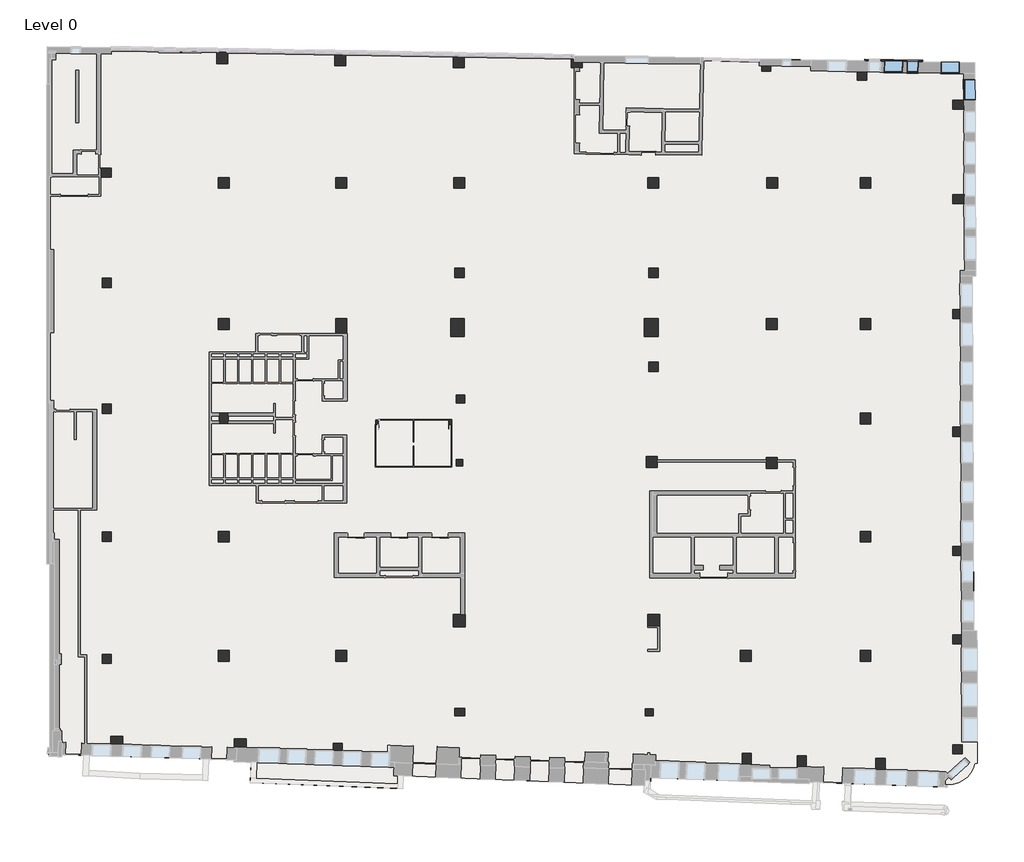
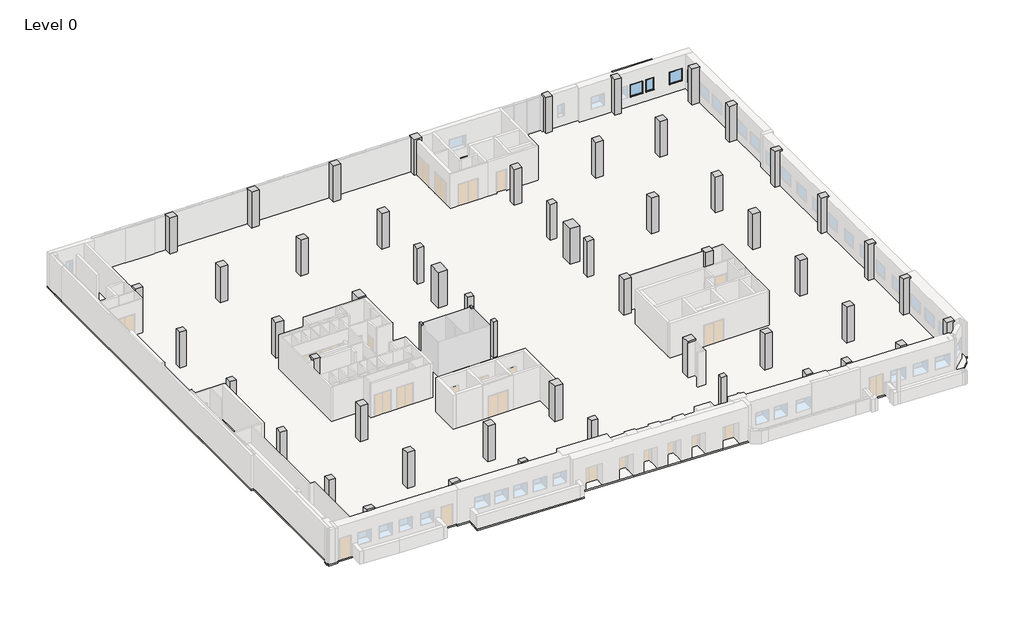
# One storey, part 9 of 9: 57 columns, 4 windows, 1 slab, 1 wall.
"""IFC4 building model written with IfcOpenShell, lengths in millimetres."""

import ifcopenshell
import ifcopenshell.guid

model = None  # the IFC model being written
_history = None  # IfcOwnerHistory: only IFC2X3 demands one
_inside = {}  # id of a spatial element -> (the spatial element, [elements in it])
_under = {}  # id of a project, library or spatial element -> (it, [spatial elements below it])
_declared = {}  # id of a project -> (the project, [libraries it declares])
_typed = {}  # id of a type object -> (the type object, [elements of that type])
_made_of = {}  # id of a material, layer set ... -> (it, [elements and type objects made of it])


def new_model(schema):
    """Start an empty IFC model of exactly this schema.

    Asked for "IFC4X3", IfcOpenShell would pick the latest addendum, in which some entities
    have other attributes; the version numbers below select the first issue.
    IFC2X3 requires an IfcOwnerHistory on every rooted entity: one is made here for all.
    """
    global model, _history
    if schema == "IFC4X3":
        model = ifcopenshell.file(schema_version=(4, 3, 0, 0))
    else:
        model = ifcopenshell.file(schema=schema)
    _inside.clear()
    _under.clear()
    _declared.clear()
    _typed.clear()
    _made_of.clear()
    _history = None
    if model.schema == "IFC2X3":
        org = make("IfcOrganization", Name="unknown")
        user = make(
            "IfcPersonAndOrganization",
            ThePerson=make("IfcPerson", FamilyName="unknown"),
            TheOrganization=org,
        )
        app = make(
            "IfcApplication",
            ApplicationDeveloper=org,
            Version="unknown",
            ApplicationFullName="unknown",
            ApplicationIdentifier="unknown",
        )
        _history = make(
            "IfcOwnerHistory",
            OwningUser=user,
            OwningApplication=app,
            ChangeAction="ADDED",
            CreationDate=0,
        )
    return model


def make(cls, **values):
    """One entity of the class cls with the attributes given. An attribute that is None is left unset."""
    return model.create_entity(
        cls, **{name: value for name, value in values.items() if value is not None}
    )


def rooted(cls, **values):
    """An entity with a GlobalId (a new one), such as an element, a storey or a relation."""
    return make(cls, GlobalId=ifcopenshell.guid.new(), OwnerHistory=_history, **values)


def si_unit(unit_type, name, prefix=None):
    """IfcSIUnit, for example si_unit("LENGTHUNIT", "METRE", prefix="MILLI")."""
    return make("IfcSIUnit", UnitType=unit_type, Prefix=prefix, Name=name)


def assignment(units):
    """IfcUnitAssignment: the units of a project."""
    return None if units is None else make("IfcUnitAssignment", Units=units)


def point(xyz):
    """IfcCartesianPoint."""
    return None if xyz is None else make("IfcCartesianPoint", Coordinates=xyz)


def direction(xyz):
    """IfcDirection."""
    return None if xyz is None else make("IfcDirection", DirectionRatios=xyz)


def frame(location, z_axis=None, x_axis=None):
    """IfcAxis2Placement3D, a coordinate frame: its origin and axes. An axis left out is left unset."""
    return make(
        "IfcAxis2Placement3D",
        Location=point(location),
        Axis=direction(z_axis),
        RefDirection=direction(x_axis),
    )


def frame_2d(location, x_axis=None):
    """IfcAxis2Placement2D, a coordinate frame in the plane: its origin and x axis."""
    return make(
        "IfcAxis2Placement2D", Location=point(location), RefDirection=direction(x_axis)
    )


def origin():
    """The frame at (0, 0, 0) with its axes left unset."""
    return frame((0.0, 0.0, 0.0))


def origin_with_axes():
    """The frame at (0, 0, 0) with the z axis (0, 0, 1) and the x axis (1, 0, 0) written out."""
    return frame((0.0, 0.0, 0.0), z_axis=(0.0, 0.0, 1.0), x_axis=(1.0, 0.0, 0.0))


def place(relative_to, where):
    """IfcLocalPlacement: puts the frame where relative to a parent placement (None: the world)."""
    return make(
        "IfcLocalPlacement", PlacementRelTo=relative_to, RelativePlacement=where
    )


def context(
    kind, dimensions, precision=None, world=None, true_north=None, identifier=None
):
    """IfcGeometricRepresentationContext, for example the 3D "Model" context."""
    return make(
        "IfcGeometricRepresentationContext",
        ContextIdentifier=identifier,
        ContextType=kind,
        CoordinateSpaceDimension=dimensions,
        Precision=precision,
        WorldCoordinateSystem=world,
        TrueNorth=true_north,
    )


def project(units=None, contexts=None):
    """IfcProject with its units and contexts."""
    return rooted(
        "IfcProject",
        Name="project",
        RepresentationContexts=contexts,
        UnitsInContext=assignment(units),
    )


def spatial(cls, under=None, at=None, **own):
    """A site, building, storey or space (cls), placed at a placement, below another one or the project."""
    s = rooted(cls, ObjectPlacement=at, **own)
    if under is not None:
        _under.setdefault(under.id(), (under, []))[1].append(s)
    return s


def polyline(points):
    """IfcPolyline through the points."""
    return make("IfcPolyline", Points=[point(p) for p in points])


def circle_curve(where, radius):
    """IfcCircle in the frame where."""
    return make("IfcCircle", Position=where, Radius=radius)


def trimmed(basis, trim1, trim2, sense, master):
    """IfcTrimmedCurve: the piece of a basis curve between two trims."""
    return make(
        "IfcTrimmedCurve",
        BasisCurve=basis,
        Trim1=trim1,
        Trim2=trim2,
        SenseAgreement=sense,
        MasterRepresentation=master,
    )


def segment(curve, same_sense, transition):
    """IfcCompositeCurveSegment."""
    return make(
        "IfcCompositeCurveSegment",
        Transition=transition,
        SameSense=same_sense,
        ParentCurve=curve,
    )


def composite_curve(segments, self_intersect=None):
    """IfcCompositeCurve: segments joined end to end."""
    return make("IfcCompositeCurve", Segments=segments, SelfIntersect=self_intersect)


def outline(outer, holes=None, kind="AREA"):
    """IfcArbitraryClosedProfileDef: a profile drawn as a closed curve; with holes, ...WithVoids."""
    if holes is None:
        return make("IfcArbitraryClosedProfileDef", ProfileType=kind, OuterCurve=outer)
    return make(
        "IfcArbitraryProfileDefWithVoids",
        ProfileType=kind,
        OuterCurve=outer,
        InnerCurves=holes,
    )


def extrude(swept, where, along, depth):
    """IfcExtrudedAreaSolid: the profile swept, set in the frame where, extruded along a direction by depth."""
    return make(
        "IfcExtrudedAreaSolid",
        SweptArea=swept,
        Position=where,
        ExtrudedDirection=direction(along),
        Depth=depth,
    )


def faces_of(points, faces, orient=None, outer=None):
    """IfcFace entities. A face is a list of loops; a loop is a list of indices into points, from 0.

    orient and outer hold one flag for each loop. By default every Orientation is true, the
    first loop of a face is its IfcFaceOuterBound and the others are IfcFaceBound.
    """
    made = []
    for i, loops in enumerate(faces):
        bounds = []
        for j, loop in enumerate(loops):
            is_outer = j == 0 if outer is None else outer[i][j]
            bounds.append(
                make(
                    "IfcFaceOuterBound" if is_outer else "IfcFaceBound",
                    Bound=make("IfcPolyLoop", Polygon=[points[k] for k in loop]),
                    Orientation=True if orient is None else orient[i][j],
                )
            )
        made.append(make("IfcFace", Bounds=bounds))
    return made


def faceted_brep(points, faces, orient=None, outer=None, voids=None):
    """IfcFacetedBrep: a solid bounded by flat faces; with voids (closed shells), ...WithVoids."""
    shared = [point(p) for p in points]
    hull = make("IfcClosedShell", CfsFaces=faces_of(shared, faces, orient, outer))
    if voids is None:
        return make("IfcFacetedBrep", Outer=hull)
    return make(
        "IfcFacetedBrepWithVoids",
        Outer=hull,
        Voids=[
            make(cls, CfsFaces=faces_of(shared, fs, o, b)) for cls, fs, o, b in voids
        ],
    )


def shape(context_of_items, identifier, shape_type, items):
    """IfcShapeRepresentation: the items that make up one representation, for example the "Body"."""
    return make(
        "IfcShapeRepresentation",
        ContextOfItems=context_of_items,
        RepresentationIdentifier=identifier,
        RepresentationType=shape_type,
        Items=items,
    )


def source(mapping_origin, context_of_items, identifier, shape_type, items):
    """IfcRepresentationMap: a shape defined once, which mapped items show again and again."""
    return make(
        "IfcRepresentationMap",
        MappingOrigin=mapping_origin,
        MappedRepresentation=shape(context_of_items, identifier, shape_type, items),
    )


def transform(
    local_origin,
    x_axis=None,
    y_axis=None,
    z_axis=None,
    scale=None,
    scale2=None,
    scale3=None,
    uniform=True,
):
    """IfcCartesianTransformationOperator3D, or its non-uniform kind. x_axis, y_axis, z_axis: its Axis1, 2, 3."""
    if uniform:
        return make(
            "IfcCartesianTransformationOperator3D",
            Axis1=direction(x_axis),
            Axis2=direction(y_axis),
            LocalOrigin=point(local_origin),
            Scale=scale,
            Axis3=direction(z_axis),
        )
    return make(
        "IfcCartesianTransformationOperator3DnonUniform",
        Axis1=direction(x_axis),
        Axis2=direction(y_axis),
        LocalOrigin=point(local_origin),
        Scale=scale,
        Axis3=direction(z_axis),
        Scale2=scale2,
        Scale3=scale3,
    )


def mapped(mapping_source, mapping_target):
    """IfcMappedItem: shows the shape of a source again, moved by a transform."""
    return make(
        "IfcMappedItem", MappingSource=mapping_source, MappingTarget=mapping_target
    )


def made_of(thing, what):
    """Note that an element or type object is made of a material, layer set ...; save() writes the relation."""
    if what is not None:
        _made_of.setdefault(what.id(), (what, []))[1].append(thing)
    return thing


def element(
    cls,
    number,
    at=None,
    inside=None,
    cuts=None,
    type_object=None,
    material=None,
    context=None,
    identifier="Body",
    shape_type=None,
    held_by="IfcProductDefinitionShape",
    body=None,
    shapes=None,
    **own,
):
    """One element of the class cls, such as IfcWall. Its Tag is "e" and its number.

    at: its placement. inside: the storey or other place that contains it. cuts: it is an
    opening in that element (IfcRelVoidsElement). A single representation is given by context,
    identifier, shape_type and body (its items); several are given by shapes. held_by: the class
    of the entity that holds the representations. save() writes the other relations.
    """
    e = rooted(cls, Tag="e%d" % number, ObjectPlacement=at, **own)
    if body is not None:
        shapes = [shape(context, identifier, shape_type, body)]
    if shapes is not None:
        e.Representation = make(held_by, Representations=shapes)
    if inside is not None:
        _inside.setdefault(inside.id(), (inside, []))[1].append(e)
    if cuts is not None:
        rooted(
            "IfcRelVoidsElement", RelatingBuildingElement=cuts, RelatedOpeningElement=e
        )
    if type_object is not None:
        _typed.setdefault(type_object.id(), (type_object, []))[1].append(e)
    return made_of(e, material)


def aggregate(whole, parts):
    """IfcRelAggregates: a whole, such as a stair, and the parts it consists of."""
    return rooted("IfcRelAggregates", RelatingObject=whole, RelatedObjects=parts)


def save(model, path):
    """Write the relations noted so far, then the file.

    IfcRelAggregates (storeys below a building ...), IfcRelContainedInSpatialStructure (elements
    in a storey), IfcRelDefinesByType, IfcRelAssociatesMaterial and IfcRelDeclares: one each for
    every whole, place, type object, material and project.
    """
    for whole, parts in _under.values():
        aggregate(whole, parts)
    for where, things in _inside.values():
        rooted(
            "IfcRelContainedInSpatialStructure",
            RelatedElements=things,
            RelatingStructure=where,
        )
    for kind, things in _typed.values():
        rooted("IfcRelDefinesByType", RelatedObjects=things, RelatingType=kind)
    for what, things in _made_of.values():
        rooted("IfcRelAssociatesMaterial", RelatedObjects=things, RelatingMaterial=what)
    for by, libraries in _declared.values():
        rooted("IfcRelDeclares", RelatingContext=by, RelatedDefinitions=libraries)
    model.write(path)


def generic_81af98c7(model_context):
    return source(origin(), model_context, "Body", "SweptSolid", [
        extrude(outline(polyline([(391.2, 387.2), (391.2, -304.8), (-304.8, -304.8), (-304.8, 387.2), (391.2, 387.2)])), origin_with_axes(), (0.0, 0.0, 1.0), 3500.0),
    ])


def window_instance_1200x1200_01b7a31e(model_context):
    return source(origin(), model_context, "Body", "SweptSolid", [
        extrude(outline(polyline([(-638.1, 377.9), (561.9, 377.9), (561.9, 352.5), (-638.1, 352.5), (-638.1, 377.9)])), frame((0.0, 0.0, 900.0), z_axis=(0.0, 0.0, 1.0), x_axis=(1.0, 0.0, 0.0)), (0.0, 0.0, 1.0), 19.05),
        extrude(outline(polyline([(498.4, 303.925), (-574.6, 303.925), (-574.6, 316.625), (498.4, 316.625), (498.4, 303.925)])), frame((0.0, 0.0, 963.5), z_axis=(0.0, 0.0, 1.0), x_axis=(1.0, 0.0, 0.0)), (0.0, 0.0, 1.0), 1073.0),
        extrude(outline(polyline([(2080.95, -619.05), (919.05, -619.05), (919.05, 542.85), (2080.95, 542.85), (2080.95, -619.05)]), holes=[polyline([(2036.5, -574.6), (2036.5, 498.4), (963.5, 498.4), (963.5, -574.6), (2036.5, -574.6)])]), frame((0.0, 288.05, 0.0), z_axis=(0.0, 1.0, 0.0), x_axis=(0.0, 0.0, 1.0)), (0.0, 0.0, 1.0), 44.45),
        extrude(outline(polyline([(2100.0, -638.1), (900.0, -638.1), (900.0, 561.9), (2100.0, 561.9), (2100.0, -638.1)]), holes=[polyline([(2068.25, -606.35), (2068.25, 530.15), (931.75, 530.15), (931.75, -606.35), (2068.25, -606.35)])]), frame((0.0, -352.5, 0.0), z_axis=(0.0, 1.0, 0.0), x_axis=(0.0, 0.0, 1.0)), (0.0, 0.0, 1.0), 640.55),
        extrude(outline(polyline([(2100.0, 561.9), (2100.0, -638.1), (900.0, -638.1), (900.0, 561.9), (2100.0, 561.9)]), holes=[polyline([(2080.95, 542.85), (919.05, 542.85), (919.05, -619.05), (2080.95, -619.05), (2080.95, 542.85)])]), frame((0.0, 288.05, 0.0), z_axis=(0.0, 1.0, 0.0), x_axis=(0.0, 0.0, 1.0)), (0.0, 0.0, 1.0), 64.45),
    ])


def window_instance_600x1200_74739665(model_context):
    return source(origin(), model_context, "Body", "SweptSolid", [
        extrude(outline(polyline([(-413.1, 377.9), (336.9, 377.9), (336.9, 352.5), (-413.1, 352.5), (-413.1, 377.9)])), frame((0.0, 0.0, 900.0), z_axis=(0.0, 0.0, 1.0), x_axis=(1.0, 0.0, 0.0)), (0.0, 0.0, 1.0), 19.05),
        extrude(outline(polyline([(273.4, 303.925), (-349.6, 303.925), (-349.6, 316.625), (273.4, 316.625), (273.4, 303.925)])), frame((0.0, 0.0, 963.5), z_axis=(0.0, 0.0, 1.0), x_axis=(1.0, 0.0, 0.0)), (0.0, 0.0, 1.0), 1073.0),
        extrude(outline(polyline([(2080.95, -394.05), (919.05, -394.05), (919.05, 317.85), (2080.95, 317.85), (2080.95, -394.05)]), holes=[polyline([(2036.5, -349.6), (2036.5, 273.4), (963.5, 273.4), (963.5, -349.6), (2036.5, -349.6)])]), frame((0.0, 288.05, 0.0), z_axis=(0.0, 1.0, 0.0), x_axis=(0.0, 0.0, 1.0)), (0.0, 0.0, 1.0), 44.45),
        extrude(outline(polyline([(2100.0, -413.1), (900.0, -413.1), (900.0, 336.9), (2100.0, 336.9), (2100.0, -413.1)]), holes=[polyline([(2068.25, -381.35), (2068.25, 305.15), (931.75, 305.15), (931.75, -381.35), (2068.25, -381.35)])]), frame((0.0, -352.5, 0.0), z_axis=(0.0, 1.0, 0.0), x_axis=(0.0, 0.0, 1.0)), (0.0, 0.0, 1.0), 640.55),
        extrude(outline(polyline([(2100.0, 336.9), (2100.0, -413.1), (900.0, -413.1), (900.0, 336.9), (2100.0, 336.9)]), holes=[polyline([(2080.95, 317.85), (919.05, 317.85), (919.05, -394.05), (2080.95, -394.05), (2080.95, 317.85)])]), frame((0.0, 288.05, 0.0), z_axis=(0.0, 1.0, 0.0), x_axis=(0.0, 0.0, 1.0)), (0.0, 0.0, 1.0), 64.45),
    ])


def window_instance_600x1200_a5f13d3b(model_context):
    return source(origin(), model_context, "Body", "SweptSolid", [
        extrude(outline(polyline([(-713.1, 377.9), (636.9, 377.9), (636.9, 352.5), (-713.1, 352.5), (-713.1, 377.9)])), frame((0.0, 0.0, 900.0), z_axis=(0.0, 0.0, 1.0), x_axis=(1.0, 0.0, 0.0)), (0.0, 0.0, 1.0), 19.05),
        extrude(outline(polyline([(573.4, 303.925), (-649.6, 303.925), (-649.6, 316.625), (573.4, 316.625), (573.4, 303.925)])), frame((0.0, 0.0, 963.5), z_axis=(0.0, 0.0, 1.0), x_axis=(1.0, 0.0, 0.0)), (0.0, 0.0, 1.0), 1073.0),
        extrude(outline(polyline([(2080.95, -694.05), (919.05, -694.05), (919.05, 617.85), (2080.95, 617.85), (2080.95, -694.05)]), holes=[polyline([(2036.5, -649.6), (2036.5, 573.4), (963.5, 573.4), (963.5, -649.6), (2036.5, -649.6)])]), frame((0.0, 288.05, 0.0), z_axis=(0.0, 1.0, 0.0), x_axis=(0.0, 0.0, 1.0)), (0.0, 0.0, 1.0), 44.45),
        extrude(outline(polyline([(2100.0, -713.1), (900.0, -713.1), (900.0, 636.9), (2100.0, 636.9), (2100.0, -713.1)]), holes=[polyline([(2068.25, -681.35), (2068.25, 605.15), (931.75, 605.15), (931.75, -681.35), (2068.25, -681.35)])]), frame((0.0, -352.5, 0.0), z_axis=(0.0, 1.0, 0.0), x_axis=(0.0, 0.0, 1.0)), (0.0, 0.0, 1.0), 640.55),
        extrude(outline(polyline([(2100.0, 636.9), (2100.0, -713.1), (900.0, -713.1), (900.0, 636.9), (2100.0, 636.9)]), holes=[polyline([(2080.95, 617.85), (919.05, 617.85), (919.05, -694.05), (2080.95, -694.05), (2080.95, 617.85)])]), frame((0.0, 288.05, 0.0), z_axis=(0.0, 1.0, 0.0), x_axis=(0.0, 0.0, 1.0)), (0.0, 0.0, 1.0), 64.45),
    ])


model = new_model("IFC4")

# Units and contexts
model_context = context("Model", 3, world=origin())
ifc_project = project(units=[si_unit("LENGTHUNIT", "METRE", prefix="MILLI")], contexts=[model_context])

# Site, building, storey
site = spatial("IfcSite", under=ifc_project)
building = spatial("IfcBuilding", under=site)
storey = spatial("IfcBuildingStorey", under=building, Name="Level 0", Elevation=0.0)

# Columns
placement = place(None, origin())
element("IfcColumn", 1, ObjectType="Generic", at=placement, inside=storey, context=model_context, shape_type="Brep", body=[
    faceted_brep([(7665.272766, 37772.5505476, 0.0), (6969.2727659, 37772.5505476, 0.0), (6969.2727659, 38457.0517549, 0.0), (7665.272766, 38444.9278709, 0.0), (7665.272766, 38487.0, 3500.0), (7665.272766, 37772.5505476, 3500.0), (7665.272766, 38444.9278709, 3350.0), (7665.272766, 38487.0, 3350.0), (6969.2727659, 37772.5505476, 3500.0), (6969.2727659, 38487.0, 3500.0), (6969.2727659, 38487.0, 3350.0), (6969.2727659, 38457.0517549, 3350.0), (7638.6893275, 38445.3909377, 900.0), (7638.6893275, 38445.3909377, 2100.0), (7038.7803372, 38455.8409765, 2100.0), (7038.7803372, 38455.8409765, 900.0), (7639.4141313, 38487.0, 900.0), (7639.4141313, 38487.0, 2100.0), (7039.3231078, 38487.0, 900.0), (7039.3231078, 38487.0, 2100.0)], [[[0, 1, 2, 3]], [[4, 5, 0, 3, 6, 7]], [[1, 0, 5, 8]], [[1, 8, 9, 10, 11, 2]], [[9, 4, 7, 10]], [[5, 4, 9, 8]], [[11, 6, 3, 2], [12, 13, 14, 15]], [[6, 11, 10, 7]], [[13, 12, 16, 17]], [[12, 15, 18, 16]], [[15, 14, 19, 18]], [[14, 13, 17, 19]], [[17, 16, 18, 19]]]),
])
element("IfcColumn", 2, ObjectType="Generic", at=placement, inside=storey, context=model_context, shape_type="Brep", body=[
    faceted_brep([(15166.0, 37643.6585068, 0.0), (14470.0, 37643.6585068, 0.0), (14470.0, 38326.3937852, 0.0), (15166.0, 38314.2699012, 0.0), (15166.0, 38335.6585068, 3500.0), (15166.0, 37643.6585068, 3500.0), (15166.0, 38314.2699012, 3350.0), (15166.0, 38335.6585068, 3350.0), (14470.0, 37643.6585068, 3500.0), (14470.0, 38335.6585068, 3500.0), (14470.0, 38335.6585068, 3350.0), (14470.0, 38326.3937852, 3350.0)], [[[0, 1, 2, 3]], [[4, 5, 0, 3, 6, 7]], [[1, 0, 5, 8]], [[1, 8, 9, 10, 11, 2]], [[9, 4, 7, 10]], [[5, 4, 9, 8]], [[11, 6, 3, 2]], [[6, 11, 10, 7]]]),
])
element("IfcColumn", 3, ObjectType="Generic", at=placement, inside=storey, context=model_context, shape_type="Brep", body=[
    faceted_brep([(22666.0, 37513.0132051, 0.0), (21970.0, 37513.0132051, 0.0), (21970.0, 38195.7484835, 0.0), (22666.0, 38183.6245995, 0.0), (22666.0, 38205.0132051, 3500.0), (22666.0, 37513.0132051, 3500.0), (22666.0, 38183.6245995, 3350.0), (22666.0, 38205.0132051, 3350.0), (21970.0, 37513.0132051, 3500.0), (21970.0, 38205.0132051, 3500.0), (21970.0, 38205.0132051, 3350.0), (21970.0, 38195.7484835, 3350.0)], [[[0, 1, 2, 3]], [[4, 5, 0, 3, 6, 7]], [[1, 0, 5, 8]], [[1, 8, 9, 10, 11, 2]], [[9, 4, 7, 10]], [[5, 4, 9, 8]], [[11, 6, 3, 2]], [[6, 11, 10, 7]]]),
])
element("IfcColumn", 4, ObjectType="Generic", at=placement, inside=storey, context=model_context, shape_type="Brep", body=[
    faceted_brep([(29464.9999959, 38185.2084834, 0.0), (29464.9999959, 38204.7657288, 0.0), (29613.8316733, 38204.7657288, 0.0), (29613.4459547, 38182.6226478, 0.0), (30160.9999959, 38204.7657288, 3500.0), (30160.9999959, 37512.7657288, 3500.0), (30160.9999959, 37512.7657288, 0.0), (30160.9999959, 37856.8987303, 0.0), (30160.9999959, 37856.8987303, 3350.0), (30160.9999959, 38204.7657288, 3350.0), (29464.9999959, 37512.7657288, 0.0), (29464.9999959, 37512.7657288, 3500.0), (29464.9999959, 38204.7657288, 3500.0), (29464.9999959, 38185.2084834, 3350.0), (29464.9999959, 38065.1902787, 3350.0), (29464.9999959, 38065.1902787, 0.0), (29613.8316733, 38204.7657288, 3350.0), (29611.355947, 38062.6408497, 3350.0), (29611.355947, 38062.6408497, 0.0), (29613.4459547, 38182.6226478, 3350.0), (29607.9398657, 37866.5326913, 0.0), (29607.9398657, 37866.5326913, 3350.0)], [[[0, 1, 2, 3]], [[4, 5, 6, 7, 8, 9]], [[10, 6, 5, 11]], [[10, 11, 12, 1, 0, 13, 14, 15]], [[1, 12, 4, 9, 16, 2]], [[5, 4, 12, 11]], [[14, 17, 18, 15]], [[17, 14, 13, 19]], [[20, 21, 8, 7]], [[21, 17, 19, 16, 9, 8]], [[21, 20, 18, 17]], [[19, 13, 0, 3]], [[6, 10, 15, 18, 20, 7]], [[16, 19, 3, 2]]]),
])
element("IfcColumn", 5, ObjectType="Generic", at=placement, inside=storey, context=model_context, shape_type="SweptSolid", body=[
    extrude(outline(polyline([(22716.0, 30551.0), (22716.0, 29859.0), (22020.0, 29859.0), (22020.0, 30551.0), (22716.0, 30551.0)])), origin_with_axes(), (0.0, 0.0, 1.0), 3500.0),
])
element("IfcColumn", 6, ObjectType="Generic", at=placement, inside=storey, context=model_context, shape_type="SweptSolid", body=[
    extrude(outline(polyline([(15216.0, 30551.0), (15216.0, 29859.0), (14520.0, 29859.0), (14520.0, 30551.0), (15216.0, 30551.0)])), origin_with_axes(), (0.0, 0.0, 1.0), 3500.0),
])
element("IfcColumn", 7, ObjectType="Generic", at=placement, inside=storey, context=model_context, shape_type="Brep", body=[
    faceted_brep([(296.0, 31151.0, 0.0), (296.0, 30559.0, 0.0), (-376.5365923, 30559.0, 0.0), (-376.5365923, 30599.0, 0.0), (-376.5365923, 30699.0, 0.0), (-389.0365923, 30699.0, 0.0), (-389.0365923, 31120.0, 0.0), (-400.0000001, 31120.0, 0.0), (-400.0000001, 31151.0, 0.0), (296.0, 31151.0, 3500.0), (296.0, 30559.0, 3500.0), (-400.0000001, 30559.0, 3500.0), (-400.0000001, 30559.0, 3350.0), (-376.5365923, 30559.0, 3350.0), (-400.0000001, 31151.0, 3500.0), (-400.0000001, 31151.0, 3350.0), (-400.0000001, 30699.0, 3350.0), (-400.0000001, 30599.0, 3350.0), (-400.0000001, 31151.0, 2100.0), (-389.0365923, 31151.0, 2100.0), (-389.0365923, 31151.0, 3350.0), (-376.5365923, 30599.0, 3350.0), (-376.5365923, 30699.0, 3350.0), (-389.0365923, 30699.0, 3350.0), (-389.0365923, 31120.0, 2100.0), (-400.0000001, 31120.0, 2100.0)], [[[0, 1, 2, 3, 4, 5, 6, 7, 8]], [[1, 0, 9, 10]], [[1, 10, 11, 12, 13, 2]], [[11, 14, 15, 16, 17, 12]], [[0, 8, 18, 19, 20, 15, 14, 9]], [[10, 9, 14, 11]], [[13, 21, 3, 2]], [[21, 13, 12, 17]], [[4, 22, 23, 5]], [[22, 21, 17, 16, 23]], [[22, 4, 3, 21]], [[24, 6, 5, 23, 20, 19]], [[20, 23, 16, 15]], [[6, 24, 25, 7]], [[24, 19, 18, 25]], [[8, 7, 25, 18]]]),
])
element("IfcColumn", 8, ObjectType="Generic", at=placement, inside=storey, context=model_context, shape_type="SweptSolid", body=[
    extrude(outline(polyline([(296.0, 24156.0), (296.0, 23564.0), (-296.0, 23564.0), (-296.0, 24156.0), (296.0, 24156.0)])), origin_with_axes(), (0.0, 0.0, 1.0), 3500.0),
])
element("IfcColumn", 9, ObjectType="Generic", at=placement, inside=storey, context=model_context, shape_type="SweptSolid", body=[
    extrude(outline(polyline([(296.0, 16171.0), (296.0, 15579.0), (-296.0, 15579.0), (-296.0, 16171.0), (296.0, 16171.0)])), origin_with_axes(), (0.0, 0.0, 1.0), 3500.0),
])
element("IfcColumn", 10, ObjectType="Generic", at=placement, inside=storey, context=model_context, shape_type="Brep", body=[
    faceted_brep([(7720.0, 15593.5000002, 0.0), (7720.0, 15593.0000002, 0.0), (7720.0, 15413.0000002, 0.0), (7720.0, 15104.5000002, 0.0), (7720.0, 14924.5000002, 0.0), (7120.0, 14924.5000002, 0.0), (7120.0, 15104.5000002, 0.0), (7120.0, 15413.0000002, 0.0), (7120.0, 15593.0000002, 0.0), (7120.0, 15593.5000002, 0.0), (7720.0, 15593.5000002, 3500.0), (7720.0, 14924.5000002, 3500.0), (7720.0, 14924.5000002, 3350.0), (7120.0, 14924.5000002, 3500.0), (7120.0, 14924.5000002, 3350.0), (7120.0, 15593.5000002, 3500.0)], [[[0, 1, 2, 3, 4, 5, 6, 7, 8, 9]], [[10, 11, 12, 4, 3, 2, 1, 0]], [[11, 13, 14, 5, 4, 12]], [[13, 15, 9, 8, 7, 6, 5, 14]], [[15, 10, 0, 9]], [[10, 15, 13, 11]]]),
])
element("IfcColumn", 11, ObjectType="Generic", at=placement, inside=storey, context=model_context, shape_type="SweptSolid", body=[
    extrude(outline(polyline([(296.0, 8051.0), (296.0, 7459.0), (-296.0, 7459.0), (-296.0, 8051.0), (296.0, 8051.0)])), origin_with_axes(), (0.0, 0.0, 1.0), 3500.0),
])
element("IfcColumn", 12, ObjectType="Generic", at=placement, inside=storey, context=model_context, shape_type="SweptSolid", body=[
    extrude(outline(polyline([(7766.0, 8101.0), (7766.0, 7409.0), (7070.0, 7409.0), (7070.0, 8101.0), (7766.0, 8101.0)])), origin_with_axes(), (0.0, 0.0, 1.0), 3500.0),
])
element("IfcColumn", 13, ObjectType="Generic", at=placement, inside=storey, context=model_context, shape_type="SweptSolid", body=[
    extrude(outline(polyline([(296.0, 296.0), (296.0, -296.0), (-296.0, -296.0), (-296.0, 296.0), (296.0, 296.0)])), origin_with_axes(), (0.0, 0.0, 1.0), 3500.0),
])
element("IfcColumn", 14, ObjectType="Generic", at=placement, inside=storey, context=model_context, shape_type="Brep", body=[
    faceted_brep([(1008.9899253, -4910.0, 0.0), (1008.9899253, -5431.2201129, 0.0), (965.7497842, -5431.2201129, 0.0), (258.9899253, -5409.7687818, 0.0), (258.9899253, -4910.0, 0.0), (1008.9899253, -4910.0, 3500.0), (1008.9899253, -5431.2201129, 3500.0), (258.9899253, -5431.2201129, 3500.0), (258.9899253, -5431.2201129, 3350.0), (965.7497842, -5431.2201129, 3350.0), (258.9899253, -4910.0, 3500.0), (258.9899253, -5409.7687818, 900.0), (258.9899253, -5431.2201129, 900.0), (258.9899253, -5431.2201129, 2100.0), (258.9899253, -5409.7687818, 2100.0), (258.9899253, -5409.7687818, 3350.0), (274.6848531, -5410.2451489, 2100.0), (274.6848531, -5410.2451489, 900.0), (274.0482282, -5431.2201129, 2100.0), (274.0482282, -5431.2201129, 900.0)], [[[0, 1, 2, 3, 4]], [[1, 0, 5, 6]], [[1, 6, 7, 8, 9, 2]], [[7, 10, 4, 3, 11, 12, 13, 14, 15, 8]], [[0, 4, 10, 5]], [[6, 5, 10, 7]], [[16, 17, 11, 3, 2, 9, 15, 14]], [[15, 9, 8]], [[17, 16, 18, 19]], [[11, 17, 19, 12]], [[16, 14, 13, 18]], [[13, 12, 19, 18]]]),
])
element("IfcColumn", 15, ObjectType="Generic", at=placement, inside=storey, context=model_context, shape_type="Brep", body=[
    faceted_brep([(8080.0, -5062.4788871, 0.0), (8830.0, -5062.4788871, 0.0), (8830.0, -5599.1439862, 0.0), (8080.0, -5571.6777079, 0.0), (8830.0, -5062.4788871, 3500.0), (8830.0, -5611.3336103, 3500.0), (8830.0, -5611.3336103, 3350.0), (8830.0, -5599.1439862, 3350.0), (8080.0, -5611.3336103, 3500.0), (8080.0, -5611.3336103, 3350.0), (8080.0, -5062.4788871, 3500.0), (8080.0, -5571.6777079, 3350.0)], [[[0, 1, 2, 3]], [[4, 5, 6, 7, 2, 1]], [[5, 8, 9, 6]], [[8, 10, 0, 3, 11, 9]], [[1, 0, 10, 4]], [[5, 4, 10, 8]], [[7, 11, 3, 2]], [[11, 7, 6, 9]]]),
])
element("IfcColumn", 16, ObjectType="Generic", at=placement, inside=storey, context=model_context, shape_type="Brep", body=[
    faceted_brep([(14943.7083494, -5367.8699587, 0.0), (14943.7083494, -5823.038406, 0.0), (14353.9588448, -5801.440774, 0.0), (14353.9588448, -5367.8699587, 0.0), (14943.7083494, -5367.8699587, 3500.0), (14943.7083494, -5823.038406, 3500.0), (14943.7083494, -5823.038406, 3350.0), (14353.9588448, -5823.038406, 3500.0), (14353.9588448, -5823.038406, 3350.0), (14353.9588448, -5367.8699587, 3500.0), (14353.9588448, -5801.440774, 900.0), (14353.9588448, -5823.038406, 900.0), (14353.9588448, -5823.038406, 2100.0), (14353.9588448, -5801.440774, 2100.0), (14353.9588448, -5801.440774, 3350.0), (14386.7917945, -5802.6431725, 2100.0), (14386.7917945, -5802.6431725, 900.0), (14386.0448863, -5823.038406, 2100.0), (14386.0448863, -5823.038406, 900.0)], [[[0, 1, 2, 3]], [[1, 0, 4, 5, 6]], [[5, 7, 8, 6]], [[7, 9, 3, 2, 10, 11, 12, 13, 14, 8]], [[0, 3, 9, 4]], [[5, 4, 9, 7]], [[15, 16, 10, 2, 1, 6, 14, 13]], [[14, 6, 8]], [[16, 15, 17, 18]], [[10, 16, 18, 11]], [[15, 13, 12, 17]], [[12, 11, 18, 17]]]),
])
element("IfcColumn", 17, ObjectType="Generic", at=placement, inside=storey, context=model_context, shape_type="SweptSolid", body=[
    extrude(outline(polyline([(22709.6531812, -3134.9932919), (22709.6531812, -3627.0183352), (22084.5, -3627.0183352), (22084.5, -3134.9932919), (22709.6531812, -3134.9932919)])), origin_with_axes(), (0.0, 0.0, 1.0), 3500.0),
])
element("IfcColumn", 18, ObjectType="Generic", at=placement, inside=storey, context=model_context, shape_type="SweptSolid", body=[
    extrude(outline(polyline([(34663.3709738, -3156.8596832), (34663.3709738, -3627.0046644), (34165.1531812, -3627.0046644), (34165.1531812, -3156.8596832), (34663.3709738, -3156.8596832)])), origin_with_axes(), (0.0, 0.0, 1.0), 3500.0),
])
element("IfcColumn", 19, ObjectType="Generic", at=placement, inside=storey, context=model_context, shape_type="SweptSolid", body=[
    extrude(outline(polyline([(48465.9999985, 551.0), (48465.9999985, -141.0), (47769.9999985, -141.0), (47769.9999985, 551.0), (48465.9999985, 551.0)])), origin_with_axes(), (0.0, 0.0, 1.0), 3500.0),
])
element("IfcColumn", 20, ObjectType="Generic", at=placement, inside=storey, context=model_context, shape_type="SweptSolid", body=[
    extrude(outline(polyline([(40880.0000014, 551.0), (40880.0000014, -141.0), (40184.0000013, -141.0), (40184.0000013, 551.0), (40880.0000014, 551.0)])), origin_with_axes(), (0.0, 0.0, 1.0), 3500.0),
])
element("IfcColumn", 21, ObjectType="Generic", at=placement, inside=storey, context=model_context, shape_type="SweptSolid", body=[
    extrude(outline(polyline([(48465.9999985, 8101.0), (48465.9999985, 7409.0), (47769.9999985, 7409.0), (47769.9999985, 8101.0), (48465.9999985, 8101.0)])), origin_with_axes(), (0.0, 0.0, 1.0), 3500.0),
])
element("IfcColumn", 22, ObjectType="Generic", at=placement, inside=storey, context=model_context, shape_type="SweptSolid", body=[
    extrude(outline(polyline([(48465.9999985, 15601.0), (48465.9999985, 14909.0), (47769.9999985, 14909.0), (47769.9999985, 15601.0), (48465.9999985, 15601.0)])), origin_with_axes(), (0.0, 0.0, 1.0), 3500.0),
])
element("IfcColumn", 23, ObjectType="Generic", at=placement, inside=storey, context=model_context, shape_type="Brep", body=[
    faceted_brep([(42507.5, 12791.0, 0.0), (42507.5, 12635.9323702, 0.0), (42507.5, 12510.9323702, 0.0), (42507.5, 12099.0, 0.0), (41811.5, 12099.0, 0.0), (41811.5, 12510.9323702, 0.0), (41824.0, 12510.9323702, 0.0), (41824.0, 12635.9323702, 0.0), (41811.5, 12635.9323702, 0.0), (41811.5, 12791.0, 0.0), (42507.5, 12791.0, 3500.0), (42507.5, 12099.0, 3500.0), (41811.5, 12099.0, 3500.0), (41811.5, 12791.0, 3500.0), (41811.5, 12635.9323702, 3350.0), (41811.5, 12510.9323702, 3350.0), (41824.0, 12635.9323702, 3350.0), (41824.0, 12510.9323702, 3350.0)], [[[0, 1, 2, 3, 4, 5, 6, 7, 8, 9]], [[3, 2, 1, 0, 10, 11]], [[4, 3, 11, 12]], [[4, 12, 13, 9, 8, 14, 15, 5]], [[0, 9, 13, 10]], [[11, 10, 13, 12]], [[7, 16, 14, 8]], [[17, 6, 5, 15]], [[16, 7, 6, 17]], [[16, 17, 15, 14]]]),
])
element("IfcColumn", 24, ObjectType="Generic", at=placement, inside=storey, context=model_context, shape_type="Brep", body=[
    faceted_brep([(22720.0, 2841.0, 0.0), (22720.0, 2025.0, 0.0), (21969.0, 2025.0, 0.0), (21969.0, 2841.0, 0.0), (22452.3210385, 2841.0, 0.0), (22702.3210385, 2841.0, 0.0), (22720.0, 2841.0, 3500.0), (22720.0, 2025.0, 3500.0), (21969.0, 2025.0, 3500.0), (21969.0, 2841.0, 3500.0)], [[[0, 1, 2, 3, 4, 5]], [[6, 7, 1, 0]], [[7, 8, 2, 1]], [[8, 9, 3, 2]], [[9, 6, 0, 5, 4, 3]], [[6, 9, 8, 7]]]),
])
element("IfcColumn", 25, ObjectType="Generic", at=placement, inside=storey, context=model_context, shape_type="SweptSolid", body=[
    extrude(outline(polyline([(15208.4826768, 551.0), (15208.4826768, -141.0), (14512.4826768, -141.0), (14512.4826768, 551.0), (15208.4826768, 551.0)])), origin_with_axes(), (0.0, 0.0, 1.0), 3500.0),
])
element("IfcColumn", 26, ObjectType="Generic", at=placement, inside=storey, context=model_context, shape_type="SweptSolid", body=[
    extrude(outline(polyline([(7766.0, 551.0), (7766.0, -141.0), (7070.0, -141.0), (7070.0, 551.0), (7766.0, 551.0)])), origin_with_axes(), (0.0, 0.0, 1.0), 3500.0),
])
element("IfcColumn", 27, ObjectType="Generic", at=placement, inside=storey, context=model_context, shape_type="SweptSolid", body=[
    extrude(outline(polyline([(7766.0, 21601.0), (7766.0, 20909.0), (7070.0, 20909.0), (7070.0, 21601.0), (7766.0, 21601.0)])), origin_with_axes(), (0.0, 0.0, 1.0), 3500.0),
])
element("IfcColumn", 28, ObjectType="Generic", at=placement, inside=storey, context=model_context, shape_type="SweptSolid", body=[
    extrude(outline(polyline([(15216.0000015, 21601.0), (15216.0000015, 20635.0000002), (14520.0000014, 20635.0000002), (14520.0000014, 21601.0), (15216.0000015, 21601.0)])), origin_with_axes(), (0.0, 0.0, 1.0), 3500.0),
])
element("IfcColumn", 29, ObjectType="Generic", at=placement, inside=storey, context=model_context, shape_type="SweptSolid", body=[
    extrude(outline(polyline([(42515.9999985, 21601.0), (42515.9999985, 20909.0), (41819.9999985, 20909.0), (41819.9999985, 21601.0), (42515.9999985, 21601.0)])), origin_with_axes(), (0.0, 0.0, 1.0), 3500.0),
])
element("IfcColumn", 30, ObjectType="Generic", at=placement, inside=storey, context=model_context, shape_type="SweptSolid", body=[
    extrude(outline(polyline([(48465.9999985, 21601.0), (48465.9999985, 20909.0), (47769.9999985, 20909.0), (47769.9999985, 21601.0), (48465.9999985, 21601.0)])), origin_with_axes(), (0.0, 0.0, 1.0), 3500.0),
])
element("IfcColumn", 31, ObjectType="Generic", at=placement, inside=storey, context=model_context, shape_type="SweptSolid", body=[
    extrude(outline(polyline([(48465.9999985, 30551.0), (48465.9999985, 29859.0), (47769.9999985, 29859.0), (47769.9999985, 30551.0), (48465.9999985, 30551.0)])), origin_with_axes(), (0.0, 0.0, 1.0), 3500.0),
])
element("IfcColumn", 32, ObjectType="Generic", at=placement, inside=storey, context=model_context, shape_type="SweptSolid", body=[
    extrude(outline(polyline([(42565.9999985, 30551.0), (42565.9999985, 29859.0), (41869.9999985, 29859.0), (41869.9999985, 30551.0), (42565.9999985, 30551.0)])), origin_with_axes(), (0.0, 0.0, 1.0), 3500.0),
])
element("IfcColumn", 33, ObjectType="Generic", at=placement, inside=storey, context=model_context, shape_type="SweptSolid", body=[
    extrude(outline(polyline([(35015.9999985, 30551.0), (35015.9999985, 29859.0), (34319.9999985, 29859.0), (34319.9999985, 30551.0), (35015.9999985, 30551.0)])), origin_with_axes(), (0.0, 0.0, 1.0), 3500.0),
])
element("IfcColumn", 34, ObjectType="Generic", at=placement, inside=storey, context=model_context, shape_type="SweptSolid", body=[
    extrude(outline(polyline([(34966.0000015, 24791.0), (34966.0000015, 24199.0), (34374.0000015, 24199.0), (34374.0000015, 24791.0), (34966.0000015, 24791.0)])), origin_with_axes(), (0.0, 0.0, 1.0), 3500.0),
])
element("IfcColumn", 35, ObjectType="Generic", at=placement, inside=storey, context=model_context, shape_type="SweptSolid", body=[
    extrude(outline(polyline([(22666.0000015, 24791.0), (22666.0000015, 24199.0), (22074.0000015, 24199.0), (22074.0000015, 24791.0), (22666.0000015, 24791.0)])), origin_with_axes(), (0.0, 0.0, 1.0), 3500.0),
])
element("IfcColumn", 36, ObjectType="Generic", at=placement, inside=storey, context=model_context, shape_type="Brep", body=[
    faceted_brep([(48192.9581475, 36722.5921858, 0.0), (47600.9581475, 36722.5921858, 0.0), (47600.9581475, 37260.8325936, 0.0), (48192.9581475, 37250.5557625, 0.0), (48192.9581475, 37414.5921858, 3500.0), (48192.9581475, 36722.5921858, 3500.0), (48192.9581475, 37250.5557625, 3350.0), (48192.9581475, 37414.5921858, 3350.0), (47600.9581475, 36722.5921858, 3500.0), (47600.9581475, 37414.5921858, 3500.0), (47600.9581475, 37414.5921858, 3350.0), (47600.9581475, 37260.8325936, 3350.0)], [[[0, 1, 2, 3]], [[4, 5, 0, 3, 6, 7]], [[1, 0, 5, 8]], [[1, 8, 9, 10, 11, 2]], [[9, 4, 7, 10]], [[5, 4, 9, 8]], [[11, 6, 3, 2]], [[6, 11, 10, 7]]]),
])
element("IfcColumn", 37, ObjectType="Generic", at=placement, inside=storey, context=model_context, shape_type="Brep", body=[
    faceted_brep([(42121.2971166, 37300.3534361, 0.0), (41529.2971137, 37300.3534361, 0.0), (41529.2971137, 37641.670407, 0.0), (42121.2971166, 37631.3581378, 0.0), (42121.2971166, 37992.3534361, 3500.0), (42121.2971166, 37300.3534361, 3500.0), (42121.2971166, 37631.3581378, 3350.0), (42121.2971166, 37992.3534361, 3350.0), (41529.2971137, 37300.3534361, 3500.0), (41529.2971137, 37992.3534361, 3500.0), (41529.2971137, 37992.3534361, 3350.0), (41529.2971137, 37641.670407, 3350.0)], [[[0, 1, 2, 3]], [[4, 5, 0, 3, 6, 7]], [[1, 0, 5, 8]], [[1, 8, 9, 10, 11, 2]], [[9, 4, 7, 10]], [[5, 4, 9, 8]], [[11, 6, 3, 2]], [[6, 11, 10, 7]]]),
])
element("IfcColumn", 38, ObjectType="Generic", at=placement, inside=storey, context=model_context, shape_type="SweptSolid", body=[
    extrude(outline(polyline([(22671.502088, 21601.0), (22671.502088, 20462.0000002), (21830.75, 20462.0000002), (21830.75, 21601.0), (22671.502088, 21601.0)])), origin_with_axes(), (0.0, 0.0, 1.0), 3500.0),
])
element("IfcColumn", 39, ObjectType="Generic", at=placement, inside=storey, context=model_context, shape_type="SweptSolid", body=[
    extrude(outline(polyline([(22692.9310385, 16746.6061446), (22692.9310385, 16247.2219366), (22161.7162432, 16247.2219366), (22161.7162432, 16746.6061446), (22692.9310385, 16746.6061446)])), origin_with_axes(), (0.0, 0.0, 1.0), 3500.0),
])
element("IfcColumn", 40, ObjectType="Generic", at=placement, inside=storey, context=model_context, shape_type="SweptSolid", body=[
    extrude(outline(polyline([(34915.3714788, 12851.7348686), (34915.3714788, 12159.7348686), (34219.3714787, 12159.7348686), (34219.3714787, 12851.7348686), (34915.3714788, 12851.7348686)])), origin_with_axes(), (0.0, 0.0, 1.0), 3500.0),
])
element("IfcColumn", 41, ObjectType="Generic", at=placement, inside=storey, context=model_context, shape_type="SweptSolid", body=[
    extrude(outline(polyline([(34966.0000015, 18851.5827576), (34966.0000015, 18224.1469875), (34374.0000014, 18224.1469875), (34374.0000014, 18851.5827576), (34966.0000015, 18851.5827576)])), origin_with_axes(), (0.0, 0.0, 1.0), 3500.0),
])
element("IfcColumn", 42, ObjectType="Generic", at=placement, inside=storey, context=model_context, shape_type="Brep", body=[
    faceted_brep([(35075.5, 2820.0, 0.0), (35075.5, 2079.0, 0.0), (34955.5, 2079.0, 0.0), (34324.0, 2079.0, 0.0), (34324.0, 2820.0, 0.0), (35075.5, 2820.0, 3500.0), (35075.5, 2079.0, 3500.0), (35075.5, 2079.0, 3350.0), (34324.0, 2079.0, 3500.0), (34324.0, 2079.0, 3350.0), (34324.0, 2820.0, 3500.0)], [[[0, 1, 2, 3, 4]], [[5, 6, 7, 1, 0]], [[6, 8, 9, 3, 2, 1, 7]], [[8, 10, 4, 3, 9]], [[10, 5, 0, 4]], [[5, 10, 8, 6]]]),
])
element("IfcColumn", 43, ObjectType="Generic", at=placement, inside=storey, context=model_context, shape_type="SweptSolid", body=[
    extrude(outline(polyline([(34966.0000015, 21601.0), (34966.0000015, 20462.0000002), (34079.2444453, 20462.0000002), (34079.2444453, 21601.0), (34966.0000015, 21601.0)])), origin_with_axes(), (0.0, 0.0, 1.0), 3500.0),
])
element("IfcColumn", 44, ObjectType="Generic", at=placement, inside=storey, context=model_context, shape_type="SweptSolid", body=[
    extrude(outline(polyline([(17221.7712719, 15174.1871925), (17221.7712719, 14890.0000002), (17052.0, 14890.0000002), (17052.0, 15174.1871925), (17221.7712719, 15174.1871925)])), origin_with_axes(), (0.0, 0.0, 1.0), 3500.0),
])
element("IfcColumn", 45, ObjectType="Generic", at=placement, inside=storey, context=model_context, shape_type="SweptSolid", body=[
    extrude(outline(polyline([(21694.0, 15186.1871925), (21873.25, 15186.1871925), (21873.25, 14890.0000002), (21694.0, 14890.0000002), (21694.0, 15186.1871925)])), origin_with_axes(), (0.0, 0.0, 1.0), 3500.0),
])
element("IfcColumn", 46, ObjectType="Generic", at=placement, inside=storey, context=model_context, shape_type="Brep", body=[
    faceted_brep([(40880.0000014, -5999.2574834, 0.0), (40880.0000014, -6684.9949076, 0.0), (40661.2576321, -6684.9949076, 0.0), (40306.4893089, -6672.0026869, 0.0), (40306.4893089, -5999.2574834, 0.0), (40880.0000014, -5999.2574834, 3500.0), (40880.0000014, -6684.9949076, 3500.0), (40306.4893089, -6684.9949076, 3500.0), (40306.4893089, -6684.9949076, 3350.0), (40661.2576321, -6684.9949076, 3350.0), (40306.4893089, -5999.2574834, 3500.0), (40306.4893089, -6672.0026869, 3350.0)], [[[0, 1, 2, 3, 4]], [[1, 0, 5, 6]], [[1, 6, 7, 8, 9, 2]], [[7, 10, 4, 3, 11, 8]], [[0, 4, 10, 5]], [[6, 5, 10, 7]], [[9, 11, 3, 2]], [[11, 9, 8]]]),
])
element("IfcColumn", 47, ObjectType="Generic", at=placement, inside=storey, context=model_context, shape_type="Brep", body=[
    faceted_brep([(43803.0, -6852.8856216, 0.0), (43803.0, -6160.8856216, 0.0), (44374.0, -6160.8856216, 0.0), (44374.0, -6842.3357352, 0.0), (43814.4747931, -6821.8449684, 0.0), (43813.3380314, -6852.8856216, 0.0), (44374.0, -6160.8856216, 3500.0), (44374.0, -6852.8856216, 3500.0), (44374.0, -6852.8856216, 3350.0), (44374.0, -6842.3357352, 3350.0), (43803.0, -6852.8856216, 3500.0), (43813.3380314, -6852.8856216, 3350.0), (43803.0, -6160.8856216, 3500.0), (43814.4747931, -6821.8449684, 3350.0)], [[[0, 1, 2, 3, 4, 5]], [[6, 7, 8, 9, 3, 2]], [[7, 10, 0, 5, 11, 8]], [[1, 0, 10, 12]], [[2, 1, 12, 6]], [[7, 6, 12, 10]], [[13, 4, 3, 9]], [[4, 13, 11, 5]], [[13, 9, 8, 11]]]),
])
element("IfcColumn", 48, ObjectType="Generic", at=placement, inside=storey, context=model_context, shape_type="Brep", body=[
    faceted_brep([(48759.5300494, -6314.1406169, 0.0), (49359.5300494, -6314.1406169, 0.0), (49359.5300494, -7024.9143433, 0.0), (48759.5300494, -7002.9413206, 0.0), (49359.5300494, -6314.1406169, 3500.0), (49359.5300494, -7026.5082428, 3500.0), (49359.5300494, -7026.5082428, 3350.0), (49359.5300494, -7024.9143433, 3350.0), (48759.5300494, -7026.5082428, 3500.0), (48759.5300494, -7026.5082428, 3350.0), (48759.5300494, -6314.1406169, 3500.0), (48759.5300494, -7002.9413206, 900.0), (48759.5300494, -7026.5082428, 900.0), (48759.5300494, -7026.5082428, 2100.0), (48759.5300494, -7002.9413206, 2100.0), (48759.5300494, -7002.9413206, 3350.0), (48763.6713569, -7003.0929824, 2100.0), (48763.6713569, -7003.0929824, 900.0), (48762.8138501, -7026.5082428, 2100.0), (48762.8138501, -7026.5082428, 900.0)], [[[0, 1, 2, 3]], [[4, 5, 6, 7, 2, 1]], [[5, 8, 9, 6]], [[8, 10, 0, 3, 11, 12, 13, 14, 15, 9]], [[1, 0, 10, 4]], [[5, 4, 10, 8]], [[16, 17, 11, 3, 2, 7, 15, 14]], [[15, 7, 6, 9]], [[17, 16, 18, 19]], [[11, 17, 19, 12]], [[16, 14, 13, 18]], [[13, 12, 19, 18]]]),
])
element("IfcColumn", 49, ObjectType="Generic", at=placement, inside=storey, context=model_context, shape_type="Brep", body=[
    faceted_brep([(53654.0, 969.9855944, 0.0), (53654.0, 1519.9855944, 0.0), (54219.3650314, 1519.9855944, 0.0), (54221.3180722, 969.9855944, 0.0), (54350.0, 1519.9855944, 3500.0), (54350.0, 969.9855944, 3500.0), (54350.0, 969.9855944, 3350.0), (54350.0, 1519.9855944, 3350.0), (53654.0, 969.9855944, 3500.0), (54221.3180722, 969.9855944, 3350.0), (53654.0, 1519.9855944, 3500.0), (54219.3650314, 1519.9855944, 3350.0)], [[[0, 1, 2, 3]], [[4, 5, 6, 7]], [[5, 8, 0, 3, 9, 6]], [[1, 0, 8, 10]], [[1, 10, 4, 7, 11, 2]], [[5, 4, 10, 8]], [[11, 9, 3, 2]], [[9, 11, 7, 6]]]),
])
element("IfcColumn", 50, ObjectType="Generic", at=placement, inside=storey, context=model_context, shape_type="Brep", body=[
    faceted_brep([(53654.0, 6555.0453859, 0.0), (53654.0, 7147.0453859, 0.0), (54195.9468152, 7147.0453859, 0.0), (54198.1968227, 6555.0453859, 0.0), (54350.0, 7147.0453859, 3500.0), (54350.0, 6555.0453859, 3500.0), (54350.0, 6555.0453859, 3350.0), (54350.0, 7147.0453859, 3350.0), (53654.0, 6555.0453859, 3500.0), (54198.1968227, 6555.0453859, 3350.0), (53654.0, 7147.0453859, 3500.0), (54195.9468152, 7147.0453859, 3350.0)], [[[0, 1, 2, 3]], [[4, 5, 6, 7]], [[5, 8, 0, 3, 9, 6]], [[1, 0, 8, 10]], [[1, 10, 4, 7, 11, 2]], [[5, 4, 10, 8]], [[11, 9, 3, 2]], [[9, 11, 7, 6]]]),
])
element("IfcColumn", 51, ObjectType="Generic", at=placement, inside=storey, context=model_context, shape_type="Brep", body=[
    faceted_brep([(53654.0, 14111.0041898, 0.0), (53654.0, 14703.0041898, 0.0), (54167.2289711, 14703.0041898, 0.0), (54169.4789785, 14111.0041898, 0.0), (54350.0, 14703.0041898, 3500.0), (54350.0, 14111.0041898, 3500.0), (54350.0, 14111.0041898, 3350.0), (54350.0, 14703.0041898, 3350.0), (53654.0, 14111.0041898, 3500.0), (54169.4789785, 14111.0041898, 3350.0), (53654.0, 14703.0041898, 3500.0), (54167.2289711, 14703.0041898, 3350.0)], [[[0, 1, 2, 3]], [[4, 5, 6, 7]], [[5, 8, 0, 3, 9, 6]], [[1, 0, 8, 10]], [[1, 10, 4, 7, 11, 2]], [[5, 4, 10, 8]], [[11, 9, 3, 2]], [[9, 11, 7, 6]]]),
])
element("IfcColumn", 52, ObjectType="Generic", at=placement, inside=storey, context=model_context, shape_type="Brep", body=[
    faceted_brep([(53654.0, 21585.9832413, 0.0), (53654.0, 22177.9832413, 0.0), (54138.8189058, 22177.9832413, 0.0), (54141.0689132, 21585.9832413, 0.0), (54350.0, 22177.9832413, 3500.0), (54350.0, 21585.9832413, 3500.0), (54350.0, 21585.9832413, 3350.0), (54350.0, 22177.9832413, 3350.0), (53654.0, 21585.9832413, 3500.0), (54141.0689132, 21585.9832413, 3350.0), (53654.0, 22177.9832413, 3500.0), (54138.8189058, 22177.9832413, 3350.0)], [[[0, 1, 2, 3]], [[4, 5, 6, 7]], [[5, 8, 0, 3, 9, 6]], [[1, 0, 8, 10]], [[1, 10, 4, 7, 11, 2]], [[5, 4, 10, 8]], [[11, 9, 3, 2]], [[9, 11, 7, 6]]]),
])
element("IfcColumn", 53, ObjectType="Generic", at=placement, inside=storey, context=model_context, shape_type="Brep", body=[
    faceted_brep([(53654.0, 28888.7867935, 0.0), (53654.0, 29474.3572804, 0.0), (54385.0792292, 29474.3572804, 0.0), (54387.3048, 28888.7867935, 0.0), (54388.699584, 29474.3572804, 3500.0), (54388.699584, 28888.7867935, 3500.0), (54388.699584, 28888.7867935, 3350.0), (54388.699584, 29474.3572804, 3350.0), (53654.0, 28888.7867935, 3500.0), (54387.3048, 28888.7867935, 3350.0), (53654.0, 29474.3572804, 3500.0), (54385.0792292, 29474.3572804, 3350.0), (54385.0792292, 29474.3572804, 2100.0), (54388.699584, 29474.3572804, 2100.0), (54388.699584, 29474.3572804, 900.0), (54385.0792292, 29474.3572804, 900.0), (54385.6342719, 29328.3198551, 900.0), (54385.6342719, 29328.3198551, 2100.0), (54388.699584, 29328.3315054, 900.0), (54388.699584, 29328.3315054, 2100.0)], [[[0, 1, 2, 3]], [[4, 5, 6, 7]], [[5, 8, 0, 3, 9, 6]], [[1, 0, 8, 10]], [[1, 10, 4, 7, 11, 12, 13, 14, 15, 2]], [[5, 4, 10, 8]], [[16, 17, 12, 11, 9, 3, 2, 15]], [[9, 11, 7, 6]], [[16, 15, 14, 18]], [[17, 16, 18, 19]], [[12, 17, 19, 13]], [[14, 13, 19, 18]]]),
])
element("IfcColumn", 54, ObjectType="Generic", at=placement, inside=storey, context=model_context, shape_type="Brep", body=[
    faceted_brep([(53654.0, 34880.432978, 0.0), (53654.0, 35466.0034648, 0.0), (54362.3068498, 35466.0034648, 0.0), (54364.5324207, 34880.432978, 0.0), (54388.699584, 35466.0034648, 3500.0), (54388.699584, 34880.432978, 3500.0), (54388.699584, 34880.432978, 3350.0), (54388.699584, 35466.0034648, 3350.0), (53654.0, 34880.432978, 3500.0), (54364.5324207, 34880.432978, 3350.0), (53654.0, 35466.0034648, 3500.0), (54362.3068498, 35466.0034648, 3350.0), (54362.3068498, 35466.0034648, 2100.0), (54388.699584, 35466.0034648, 2100.0), (54388.699584, 35466.0034648, 900.0), (54362.3068498, 35466.0034648, 900.0), (54362.393231, 35443.2756893, 900.0), (54362.393231, 35443.2756893, 2100.0), (54388.699584, 35443.3756716, 900.0), (54388.699584, 35443.3756716, 2100.0)], [[[0, 1, 2, 3]], [[4, 5, 6, 7]], [[5, 8, 0, 3, 9, 6]], [[1, 0, 8, 10]], [[1, 10, 4, 7, 11, 12, 13, 14, 15, 2]], [[5, 4, 10, 8]], [[16, 17, 12, 11, 9, 3, 2, 15]], [[9, 11, 7, 6]], [[16, 15, 14, 18]], [[17, 16, 18, 19]], [[12, 17, 19, 13]], [[14, 13, 19, 18]]]),
])
element("IfcColumn", 55, ObjectType="Generic", at=placement, inside=storey, context=model_context, shape_type="Brep", body=[
    faceted_brep([(53654.0, -6019.8164224, 0.0), (53654.0, -5448.4662985, 0.0), (54244.1098877, -5448.4662985, 0.0), (54246.1387425, -6019.8164224, 0.0), (54350.0, -5448.4662985, 3500.0), (54350.0, -6019.8164224, 3500.0), (54350.0, -6019.8164224, 3350.0), (54350.0, -5448.4662985, 3350.0), (53654.0, -6019.8164224, 3500.0), (54246.1387425, -6019.8164224, 3350.0), (53654.0, -5448.4662985, 3500.0), (54244.1098877, -5448.4662985, 3350.0)], [[[0, 1, 2, 3]], [[4, 5, 6, 7]], [[5, 8, 0, 3, 9, 6]], [[1, 0, 8, 10]], [[1, 10, 4, 7, 11, 2]], [[5, 4, 10, 8]], [[11, 9, 3, 2]], [[9, 11, 7, 6]]]),
])
element("IfcColumn", 56, ObjectType="Generic", at=placement, inside=storey, context=model_context, shape_type="SweptSolid", body=[
    extrude(outline(polyline([(22170.543509, 12645.4323702), (22570.543509, 12645.4323702), (22570.543509, 12245.4323702), (22170.543509, 12245.4323702), (22170.543509, 12645.4323702)])), origin_with_axes(), (0.0, 0.0, 1.0), 3500.0),
])
generic_shape = generic_81af98c7(model_context)
element("IfcColumn", 57, ObjectType="Generic", at=placement, inside=storey, context=model_context, shape_type="MappedRepresentation", body=[
    mapped(generic_shape, transform((7374.8, 30163.8, 0.0), x_axis=(1.0, 0.0, 0.0), y_axis=(0.0, 1.0, 0.0), z_axis=(0.0, 0.0, 1.0))),
])

# Slab
element("IfcSlab", 58, at=placement, inside=storey, context=model_context, shape_type="SweptSolid", body=[
    extrude(outline(composite_curve([segment(polyline([(-3777.3699784, 38850.8384146), (298.4009598, 38779.8410381), (299.8054816, 38860.4709085), (29616.3579911, 38349.7949288), (29615.2548929, 38286.4689846), (37854.3546331, 38142.9490284), (37854.0393738, 38125.4548993), (48072.0754153, 37957.7604465), (48073.5392534, 38042.0852879), (51753.7294063, 37978.1989843), (51752.2655682, 37893.8741413), (55058.3024881, 37836.4829537), (55109.7275006, 24306.0356143), (54890.7394945, 24305.2033091), (54976.3496388, 1780.2978526), (55188.4441081, 1781.0509965), (55218.2485271, -6612.235169), (55052.9615963, -6612.8221001)]), True, "CONTINUOUS"), segment(trimmed(circle_curve(frame_2d((53349.1533898, -6253.2469608)), 1741.3376139), [point((55052.9615963, -6612.8221001))], [point((53316.8362932, -7994.2846659))], False, "CARTESIAN"), True, "CONTINUOUS"), segment(polyline([(53316.8362932, -7994.2846659), (53316.8362932, -8140.4878826), (44543.4451089, -7819.1913433), (44539.9664478, -7914.1803963), (34483.8382747, -7544.494611), (34481.9366141, -8051.3878571), (18818.2079633, -7430.2640607), (18775.9428821, -8237.7945827), (9110.1095516, -7860.6438953), (9162.6802007, -6561.9641346), (8038.7698306, -6520.8046213), (8042.9604329, -6406.37515), (-2858.3577422, -6075.5021064), (-2864.6531949, -6219.9572237), (-3668.1176738, -6193.325367), (-3663.9069079, -6025.2361443), (-3785.7915102, -6025.2361443), (-3756.3730511, -5642.8530784), (-3600.9161261, -5642.8530784), (-3600.9161261, 6016.8715147), (-3819.3638329, 6016.8715147), (-3819.3638329, 36458.37601), (-3777.3699784, 36458.37601), (-3777.3699784, 38850.8384146)]), True, "CONTINUOUS")], self_intersect=False)), frame((0.0, 0.0, -150.0), z_axis=(0.0, 0.0, 1.0), x_axis=(1.0, 0.0, 0.0)), (0.0, 0.0, 1.0), 150.0),
])

# Wall
element("IfcWall", 59, at=placement, inside=storey, context=model_context, shape_type="Brep", body=[
    faceted_brep([(51753.7294063, 37978.1989843, 0.0), (48073.5392534, 38042.0852879, 0.0), (48073.5392534, 38042.0852879, 3350.0), (51753.7294063, 37978.1989843, 3350.0), (49074.2456392, 38024.7135138, 2100.0), (48318.502346, 38037.8328483, 2100.0), (48318.502346, 38037.8328483, 900.0), (49074.2456392, 38024.7135138, 900.0), (49299.2117447, 38020.8082121, 2100.0), (49299.2117447, 38020.8082121, 900.0), (50499.030974, 37999.9799363, 900.0), (50499.030974, 37999.9799363, 2100.0), (50738.8823083, 37995.8162343, 2100.0), (50738.8823083, 37995.8162343, 900.0), (51488.7693266, 37982.7985619, 900.0), (51488.7693266, 37982.7985619, 2100.0), (48071.6299948, 37932.1018586, 0.0), (51751.8201477, 37868.215555, 0.0), (51751.8201477, 37868.215555, 3350.0), (48071.6299948, 37932.1018586, 3350.0), (49072.3363805, 37914.7300845, 900.0), (48316.5930874, 37927.8494189, 900.0), (48316.5930874, 37927.8494189, 2100.0), (49072.3363805, 37914.7300845, 2100.0), (49297.302486, 37910.8247828, 2100.0), (50497.1217153, 37889.996507, 2100.0), (50497.1217153, 37889.996507, 900.0), (49297.302486, 37910.8247828, 900.0), (50736.9730496, 37885.832805, 2100.0), (51486.8600679, 37872.8151326, 2100.0), (51486.8600679, 37872.8151326, 900.0), (50736.9730496, 37885.832805, 900.0), (51752.2655682, 37893.8741413, 0.0), (48072.0754153, 37957.7604465, 0.0), (48072.0754153, 37957.7604465, 3350.0), (51752.2655682, 37893.8741413, 3350.0)], [[[0, 1, 2, 3], [4, 5, 6, 7], [8, 9, 10, 11], [12, 13, 14, 15]], [[16, 17, 18, 19], [20, 21, 22, 23], [24, 25, 26, 27], [28, 29, 30, 31]], [[1, 0, 32, 17, 16, 33]], [[2, 1, 33, 16, 19, 34]], [[3, 2, 34, 19, 18, 35]], [[0, 3, 35, 18, 17, 32]], [[6, 21, 20, 7]], [[22, 21, 6, 5]], [[22, 5, 4, 23]], [[7, 20, 23, 4]], [[9, 8, 24, 27]], [[10, 9, 27, 26]], [[11, 10, 26, 25]], [[8, 11, 25, 24]], [[13, 12, 28, 31]], [[14, 13, 31, 30]], [[15, 14, 30, 29]], [[12, 15, 29, 28]]]),
])

# Windows
window_instance_1200x1200_shape = window_instance_1200x1200_01b7a31e(model_context)
element("IfcWindow", 60, ObjectType="Window-Instance : 1200x1200", at=placement, inside=storey, context=model_context, shape_type="MappedRepresentation", body=[
    mapped(window_instance_1200x1200_shape, transform((49853.4449545, 37574.2836312, 0.0), x_axis=(-0.9998493577177447, 0.017356896940795855, 0.0), y_axis=(-0.017356896940795855, -0.9998493577177447, 0.0), z_axis=(0.0, 0.0, 1.0))),
])
window_instance_600x1200_shape = window_instance_600x1200_74739665(model_context)
element("IfcWindow", 61, ObjectType="Window-Instance : 600x1200", at=placement, inside=storey, context=model_context, shape_type="MappedRepresentation", body=[
    mapped(window_instance_600x1200_shape, transform((51068.1494126, 37553.1969546, 0.0), x_axis=(-0.9998493577177447, 0.017356896940795855, 0.0), y_axis=(-0.017356896940795855, -0.9998493577177447, 0.0), z_axis=(0.0, 0.0, 1.0))),
])
element("IfcWindow", 62, ObjectType="Window-Instance : 600x1200", at=placement, inside=storey, context=model_context, shape_type="MappedRepresentation", body=[
    mapped(window_instance_1200x1200_shape, transform((53447.790884, 37511.8875398, 0.0), x_axis=(-0.9998493577177447, 0.017356896940795855, 0.0), y_axis=(-0.017356896940795855, -0.9998493577177447, 0.0), z_axis=(0.0, 0.0, 1.0))),
])
window_instance_600x1200_2_shape = window_instance_600x1200_a5f13d3b(model_context)
element("IfcWindow", 63, ObjectType="Window-Instance : 600x1200", at=placement, inside=storey, context=model_context, shape_type="MappedRepresentation", body=[
    mapped(window_instance_600x1200_2_shape, transform((54712.1804338, 36157.7102719, 0.0), x_axis=(-0.0038006608193690565, 0.9999927774625855, 0.0), y_axis=(-0.9999927774625855, -0.0038006608193690565, 0.0), z_axis=(0.0, 0.0, 1.0))),
])

save(model, "model.ifc")

# Revit data of these elements
# Type "WWm-ConcreteRectangular-Instance : Generic"
#   Depth [instance default] = 600 mm
#   Offset Base = 0 mm
#   Offset Top = 0 mm
#   Width [instance default] = 600 mm
